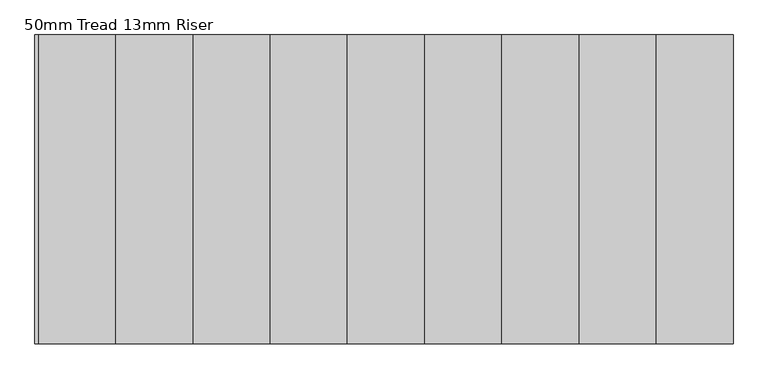
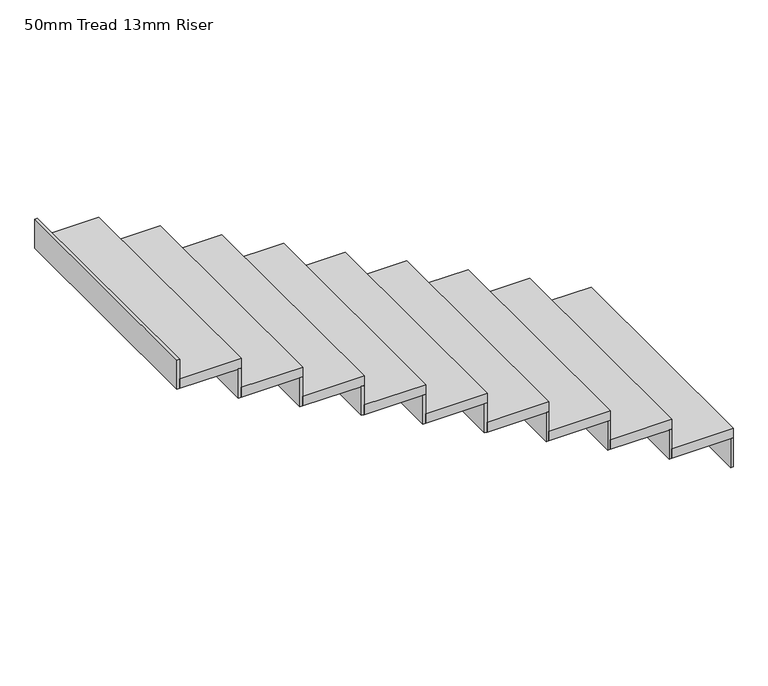
"""IFC4 building model written with IfcOpenShell, lengths in millimetres: stair flight geometry, 50mm Tread 13mm Riser."""

import ifcopenshell
import ifcopenshell.guid

model = None  # the IFC model being written
_history = None  # IfcOwnerHistory: only IFC2X3 demands one
_inside = {}  # id of a spatial element -> (the spatial element, [elements in it])
_under = {}  # id of a project, library or spatial element -> (it, [spatial elements below it])
_declared = {}  # id of a project -> (the project, [libraries it declares])
_typed = {}  # id of a type object -> (the type object, [elements of that type])
_made_of = {}  # id of a material, layer set ... -> (it, [elements and type objects made of it])


def new_model(schema):
    """Start an empty IFC model of exactly this schema.

    Asked for "IFC4X3", IfcOpenShell would pick the latest addendum, in which some entities
    have other attributes; the version numbers below select the first issue.
    IFC2X3 requires an IfcOwnerHistory on every rooted entity: one is made here for all.
    """
    global model, _history
    if schema == "IFC4X3":
        model = ifcopenshell.file(schema_version=(4, 3, 0, 0))
    else:
        model = ifcopenshell.file(schema=schema)
    _inside.clear()
    _under.clear()
    _declared.clear()
    _typed.clear()
    _made_of.clear()
    _history = None
    if model.schema == "IFC2X3":
        org = make("IfcOrganization", Name="unknown")
        user = make(
            "IfcPersonAndOrganization",
            ThePerson=make("IfcPerson", FamilyName="unknown"),
            TheOrganization=org,
        )
        app = make(
            "IfcApplication",
            ApplicationDeveloper=org,
            Version="unknown",
            ApplicationFullName="unknown",
            ApplicationIdentifier="unknown",
        )
        _history = make(
            "IfcOwnerHistory",
            OwningUser=user,
            OwningApplication=app,
            ChangeAction="ADDED",
            CreationDate=0,
        )
    return model


def make(cls, **values):
    """One entity of the class cls with the attributes given. An attribute that is None is left unset."""
    return model.create_entity(
        cls, **{name: value for name, value in values.items() if value is not None}
    )


def rooted(cls, **values):
    """An entity with a GlobalId (a new one), such as an element, a storey or a relation."""
    return make(cls, GlobalId=ifcopenshell.guid.new(), OwnerHistory=_history, **values)


def si_unit(unit_type, name, prefix=None):
    """IfcSIUnit, for example si_unit("LENGTHUNIT", "METRE", prefix="MILLI")."""
    return make("IfcSIUnit", UnitType=unit_type, Prefix=prefix, Name=name)


def assignment(units):
    """IfcUnitAssignment: the units of a project."""
    return None if units is None else make("IfcUnitAssignment", Units=units)


def point(xyz):
    """IfcCartesianPoint."""
    return None if xyz is None else make("IfcCartesianPoint", Coordinates=xyz)


def direction(xyz):
    """IfcDirection."""
    return None if xyz is None else make("IfcDirection", DirectionRatios=xyz)


def frame(location, z_axis=None, x_axis=None):
    """IfcAxis2Placement3D, a coordinate frame: its origin and axes. An axis left out is left unset."""
    return make(
        "IfcAxis2Placement3D",
        Location=point(location),
        Axis=direction(z_axis),
        RefDirection=direction(x_axis),
    )


def origin():
    """The frame at (0, 0, 0) with its axes left unset."""
    return frame((0.0, 0.0, 0.0))


def place(relative_to, where):
    """IfcLocalPlacement: puts the frame where relative to a parent placement (None: the world)."""
    return make(
        "IfcLocalPlacement", PlacementRelTo=relative_to, RelativePlacement=where
    )


def context(
    kind, dimensions, precision=None, world=None, true_north=None, identifier=None
):
    """IfcGeometricRepresentationContext, for example the 3D "Model" context."""
    return make(
        "IfcGeometricRepresentationContext",
        ContextIdentifier=identifier,
        ContextType=kind,
        CoordinateSpaceDimension=dimensions,
        Precision=precision,
        WorldCoordinateSystem=world,
        TrueNorth=true_north,
    )


def project(units=None, contexts=None):
    """IfcProject with its units and contexts."""
    return rooted(
        "IfcProject",
        Name="project",
        RepresentationContexts=contexts,
        UnitsInContext=assignment(units),
    )


def spatial(cls, under=None, at=None, **own):
    """A site, building, storey or space (cls), placed at a placement, below another one or the project."""
    s = rooted(cls, ObjectPlacement=at, **own)
    if under is not None:
        _under.setdefault(under.id(), (under, []))[1].append(s)
    return s


def polyline(points):
    """IfcPolyline through the points."""
    return make("IfcPolyline", Points=[point(p) for p in points])


def outline(outer, holes=None, kind="AREA"):
    """IfcArbitraryClosedProfileDef: a profile drawn as a closed curve; with holes, ...WithVoids."""
    if holes is None:
        return make("IfcArbitraryClosedProfileDef", ProfileType=kind, OuterCurve=outer)
    return make(
        "IfcArbitraryProfileDefWithVoids",
        ProfileType=kind,
        OuterCurve=outer,
        InnerCurves=holes,
    )


def extrude(swept, where, along, depth):
    """IfcExtrudedAreaSolid: the profile swept, set in the frame where, extruded along a direction by depth."""
    return make(
        "IfcExtrudedAreaSolid",
        SweptArea=swept,
        Position=where,
        ExtrudedDirection=direction(along),
        Depth=depth,
    )


def shape(context_of_items, identifier, shape_type, items):
    """IfcShapeRepresentation: the items that make up one representation, for example the "Body"."""
    return make(
        "IfcShapeRepresentation",
        ContextOfItems=context_of_items,
        RepresentationIdentifier=identifier,
        RepresentationType=shape_type,
        Items=items,
    )


def source(mapping_origin, context_of_items, identifier, shape_type, items):
    """IfcRepresentationMap: a shape defined once, which mapped items show again and again."""
    return make(
        "IfcRepresentationMap",
        MappingOrigin=mapping_origin,
        MappedRepresentation=shape(context_of_items, identifier, shape_type, items),
    )


def transform(
    local_origin,
    x_axis=None,
    y_axis=None,
    z_axis=None,
    scale=None,
    scale2=None,
    scale3=None,
    uniform=True,
):
    """IfcCartesianTransformationOperator3D, or its non-uniform kind. x_axis, y_axis, z_axis: its Axis1, 2, 3."""
    if uniform:
        return make(
            "IfcCartesianTransformationOperator3D",
            Axis1=direction(x_axis),
            Axis2=direction(y_axis),
            LocalOrigin=point(local_origin),
            Scale=scale,
            Axis3=direction(z_axis),
        )
    return make(
        "IfcCartesianTransformationOperator3DnonUniform",
        Axis1=direction(x_axis),
        Axis2=direction(y_axis),
        LocalOrigin=point(local_origin),
        Scale=scale,
        Axis3=direction(z_axis),
        Scale2=scale2,
        Scale3=scale3,
    )


def mapped(mapping_source, mapping_target):
    """IfcMappedItem: shows the shape of a source again, moved by a transform."""
    return make(
        "IfcMappedItem", MappingSource=mapping_source, MappingTarget=mapping_target
    )


def made_of(thing, what):
    """Note that an element or type object is made of a material, layer set ...; save() writes the relation."""
    if what is not None:
        _made_of.setdefault(what.id(), (what, []))[1].append(thing)
    return thing


def element(
    cls,
    number,
    at=None,
    inside=None,
    cuts=None,
    type_object=None,
    material=None,
    context=None,
    identifier="Body",
    shape_type=None,
    held_by="IfcProductDefinitionShape",
    body=None,
    shapes=None,
    **own,
):
    """One element of the class cls, such as IfcWall. Its Tag is "e" and its number.

    at: its placement. inside: the storey or other place that contains it. cuts: it is an
    opening in that element (IfcRelVoidsElement). A single representation is given by context,
    identifier, shape_type and body (its items); several are given by shapes. held_by: the class
    of the entity that holds the representations. save() writes the other relations.
    """
    e = rooted(cls, Tag="e%d" % number, ObjectPlacement=at, **own)
    if body is not None:
        shapes = [shape(context, identifier, shape_type, body)]
    if shapes is not None:
        e.Representation = make(held_by, Representations=shapes)
    if inside is not None:
        _inside.setdefault(inside.id(), (inside, []))[1].append(e)
    if cuts is not None:
        rooted(
            "IfcRelVoidsElement", RelatingBuildingElement=cuts, RelatedOpeningElement=e
        )
    if type_object is not None:
        _typed.setdefault(type_object.id(), (type_object, []))[1].append(e)
    return made_of(e, material)


def aggregate(whole, parts):
    """IfcRelAggregates: a whole, such as a stair, and the parts it consists of."""
    return rooted("IfcRelAggregates", RelatingObject=whole, RelatedObjects=parts)


def save(model, path):
    """Write the relations noted so far, then the file.

    IfcRelAggregates (storeys below a building ...), IfcRelContainedInSpatialStructure (elements
    in a storey), IfcRelDefinesByType, IfcRelAssociatesMaterial and IfcRelDeclares: one each for
    every whole, place, type object, material and project.
    """
    for whole, parts in _under.values():
        aggregate(whole, parts)
    for where, things in _inside.values():
        rooted(
            "IfcRelContainedInSpatialStructure",
            RelatedElements=things,
            RelatingStructure=where,
        )
    for kind, things in _typed.values():
        rooted("IfcRelDefinesByType", RelatedObjects=things, RelatingType=kind)
    for what, things in _made_of.values():
        rooted("IfcRelAssociatesMaterial", RelatedObjects=things, RelatingMaterial=what)
    for by, libraries in _declared.values():
        rooted("IfcRelDeclares", RelatingContext=by, RelatedDefinitions=libraries)
    model.write(path)


def stair_flight_50mm_tread_13mm_riser_8c888114(model_context):
    return source(origin(), model_context, "Body", "SweptSolid", [
        extrude(outline(polyline([(18637.0372571, -4900.9614996), (18649.5372571, -4900.9614996), (18649.5372571, -6100.9614996), (18637.0372571, -6100.9614996), (18637.0372571, -4900.9614996)])), frame((0.0, 0.0, 1450.0), z_axis=(0.0, 0.0, 1.0), x_axis=(1.0, 0.0, 0.0)), (0.0, 0.0, 1.0), 150.0),
        extrude(outline(polyline([(18349.5372571, -6100.9614996), (18349.5372571, -4900.9614996), (18649.5372571, -4900.9614996), (18649.5372571, -6100.9614996), (18349.5372571, -6100.9614996)])), frame((0.0, 0.0, 1600.0), z_axis=(0.0, 0.0, 1.0), x_axis=(1.0, 0.0, 0.0)), (0.0, 0.0, 1.0), 50.0),
        extrude(outline(polyline([(18337.0372571, -4900.9614996), (18349.5372571, -4900.9614996), (18349.5372571, -6100.9614996), (18337.0372571, -6100.9614996), (18337.0372571, -4900.9614996)])), frame((0.0, 0.0, 1600.0), z_axis=(0.0, 0.0, 1.0), x_axis=(1.0, 0.0, 0.0)), (0.0, 0.0, 1.0), 150.0),
        extrude(outline(polyline([(18049.5372571, -6100.9614996), (18049.5372571, -4900.9614996), (18349.5372571, -4900.9614996), (18349.5372571, -6100.9614996), (18049.5372571, -6100.9614996)])), frame((0.0, 0.0, 1750.0), z_axis=(0.0, 0.0, 1.0), x_axis=(1.0, 0.0, 0.0)), (0.0, 0.0, 1.0), 50.0),
        extrude(outline(polyline([(18037.0372571, -4900.9614996), (18049.5372571, -4900.9614996), (18049.5372571, -6100.9614996), (18037.0372571, -6100.9614996), (18037.0372571, -4900.9614996)])), frame((0.0, 0.0, 1750.0), z_axis=(0.0, 0.0, 1.0), x_axis=(1.0, 0.0, 0.0)), (0.0, 0.0, 1.0), 150.0),
        extrude(outline(polyline([(17749.5372571, -6100.9614996), (17749.5372571, -4900.9614996), (18049.5372571, -4900.9614996), (18049.5372571, -6100.9614996), (17749.5372571, -6100.9614996)])), frame((0.0, 0.0, 1900.0), z_axis=(0.0, 0.0, 1.0), x_axis=(1.0, 0.0, 0.0)), (0.0, 0.0, 1.0), 50.0),
        extrude(outline(polyline([(17737.0372571, -4900.9614996), (17749.5372571, -4900.9614996), (17749.5372571, -6100.9614996), (17737.0372571, -6100.9614996), (17737.0372571, -4900.9614996)])), frame((0.0, 0.0, 1900.0), z_axis=(0.0, 0.0, 1.0), x_axis=(1.0, 0.0, 0.0)), (0.0, 0.0, 1.0), 150.0),
        extrude(outline(polyline([(17449.5372571, -6100.9614996), (17449.5372571, -4900.9614996), (17749.5372571, -4900.9614996), (17749.5372571, -6100.9614996), (17449.5372571, -6100.9614996)])), frame((0.0, 0.0, 2050.0), z_axis=(0.0, 0.0, 1.0), x_axis=(1.0, 0.0, 0.0)), (0.0, 0.0, 1.0), 50.0),
        extrude(outline(polyline([(17437.0372571, -4900.9614996), (17449.5372571, -4900.9614996), (17449.5372571, -6100.9614996), (17437.0372571, -6100.9614996), (17437.0372571, -4900.9614996)])), frame((0.0, 0.0, 2050.0), z_axis=(0.0, 0.0, 1.0), x_axis=(1.0, 0.0, 0.0)), (0.0, 0.0, 1.0), 150.0),
        extrude(outline(polyline([(17149.5372571, -6100.9614996), (17149.5372571, -4900.9614996), (17449.5372571, -4900.9614996), (17449.5372571, -6100.9614996), (17149.5372571, -6100.9614996)])), frame((0.0, 0.0, 2200.0), z_axis=(0.0, 0.0, 1.0), x_axis=(1.0, 0.0, 0.0)), (0.0, 0.0, 1.0), 50.0),
        extrude(outline(polyline([(17137.0372571, -4900.9614996), (17149.5372571, -4900.9614996), (17149.5372571, -6100.9614996), (17137.0372571, -6100.9614996), (17137.0372571, -4900.9614996)])), frame((0.0, 0.0, 2200.0), z_axis=(0.0, 0.0, 1.0), x_axis=(1.0, 0.0, 0.0)), (0.0, 0.0, 1.0), 150.0),
        extrude(outline(polyline([(16849.5372571, -6100.9614996), (16849.5372571, -4900.9614996), (17149.5372571, -4900.9614996), (17149.5372571, -6100.9614996), (16849.5372571, -6100.9614996)])), frame((0.0, 0.0, 2350.0), z_axis=(0.0, 0.0, 1.0), x_axis=(1.0, 0.0, 0.0)), (0.0, 0.0, 1.0), 50.0),
        extrude(outline(polyline([(16837.0372571, -4900.9614996), (16849.5372571, -4900.9614996), (16849.5372571, -6100.9614996), (16837.0372571, -6100.9614996), (16837.0372571, -4900.9614996)])), frame((0.0, 0.0, 2350.0), z_axis=(0.0, 0.0, 1.0), x_axis=(1.0, 0.0, 0.0)), (0.0, 0.0, 1.0), 150.0),
        extrude(outline(polyline([(16549.5372571, -6100.9614996), (16549.5372571, -4900.9614996), (16849.5372571, -4900.9614996), (16849.5372571, -6100.9614996), (16549.5372571, -6100.9614996)])), frame((0.0, 0.0, 2500.0), z_axis=(0.0, 0.0, 1.0), x_axis=(1.0, 0.0, 0.0)), (0.0, 0.0, 1.0), 50.0),
        extrude(outline(polyline([(16537.0372571, -4900.9614996), (16549.5372571, -4900.9614996), (16549.5372571, -6100.9614996), (16537.0372571, -6100.9614996), (16537.0372571, -4900.9614996)])), frame((0.0, 0.0, 2500.0), z_axis=(0.0, 0.0, 1.0), x_axis=(1.0, 0.0, 0.0)), (0.0, 0.0, 1.0), 150.0),
        extrude(outline(polyline([(16249.5372571, -6100.9614996), (16249.5372571, -4900.9614996), (16549.5372571, -4900.9614996), (16549.5372571, -6100.9614996), (16249.5372571, -6100.9614996)])), frame((0.0, 0.0, 2650.0), z_axis=(0.0, 0.0, 1.0), x_axis=(1.0, 0.0, 0.0)), (0.0, 0.0, 1.0), 50.0),
        extrude(outline(polyline([(16237.0372571, -4900.9614996), (16249.5372571, -4900.9614996), (16249.5372571, -6100.9614996), (16237.0372571, -6100.9614996), (16237.0372571, -4900.9614996)])), frame((0.0, 0.0, 2650.0), z_axis=(0.0, 0.0, 1.0), x_axis=(1.0, 0.0, 0.0)), (0.0, 0.0, 1.0), 150.0),
        extrude(outline(polyline([(15937.0372571, -4900.9614996), (15949.5372571, -4900.9614996), (15949.5372571, -6100.9614996), (15937.0372571, -6100.9614996), (15937.0372571, -4900.9614996)])), frame((0.0, 0.0, 2800.0), z_axis=(0.0, 0.0, 1.0), x_axis=(1.0, 0.0, 0.0)), (0.0, 0.0, 1.0), 150.0),
        extrude(outline(polyline([(15949.5372571, -6100.9614996), (15949.5372571, -4900.9614996), (16249.5372571, -4900.9614996), (16249.5372571, -6100.9614996), (15949.5372571, -6100.9614996)])), frame((0.0, 0.0, 2800.0), z_axis=(0.0, 0.0, 1.0), x_axis=(1.0, 0.0, 0.0)), (0.0, 0.0, 1.0), 50.0),
    ])


if __name__ == "__main__":
    model = new_model("IFC4")
    model_context = context("Model", 3, world=origin())
    ifc_project = project(units=[si_unit("LENGTHUNIT", "METRE", prefix="MILLI")], contexts=[model_context])
    site = spatial("IfcSite", under=ifc_project)
    building = spatial("IfcBuilding", under=site)
    placement = place(None, origin())
    stair_flight_50mm_tread_13mm_riser_shape = stair_flight_50mm_tread_13mm_riser_8c888114(model_context)
    element("IfcStairFlight", 1, ObjectType="50mm Tread 13mm Riser", at=placement, inside=building, context=model_context, shape_type="MappedRepresentation", body=[
        mapped(stair_flight_50mm_tread_13mm_riser_shape, transform((0.0, 0.0, 0.0), x_axis=(1.0, 0.0, 0.0), y_axis=(0.0, 1.0, 0.0), z_axis=(0.0, 0.0, 1.0))),
    ])
    save(model, "model.ifc")
